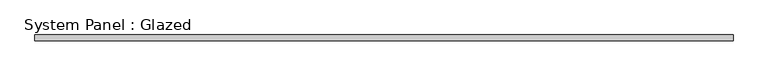
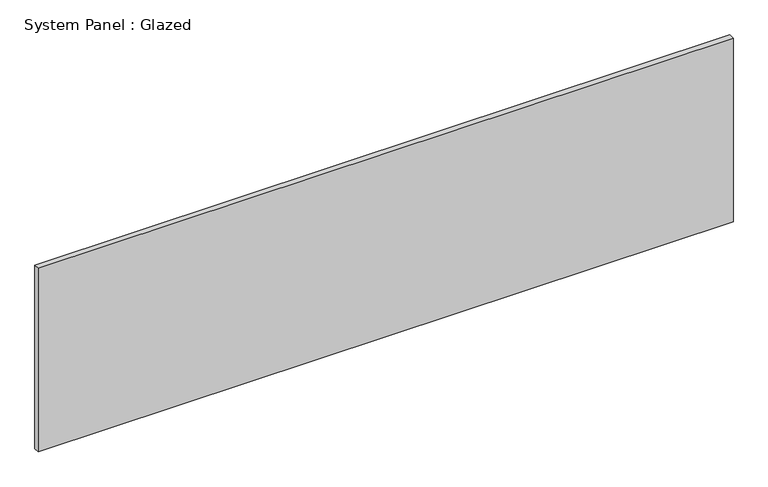
"""IFC4 building model written with IfcOpenShell, lengths in millimetres: plate geometry, System Panel : Glazed."""

import ifcopenshell
import ifcopenshell.guid

model = None  # the IFC model being written
_history = None  # IfcOwnerHistory: only IFC2X3 demands one
_inside = {}  # id of a spatial element -> (the spatial element, [elements in it])
_under = {}  # id of a project, library or spatial element -> (it, [spatial elements below it])
_declared = {}  # id of a project -> (the project, [libraries it declares])
_typed = {}  # id of a type object -> (the type object, [elements of that type])
_made_of = {}  # id of a material, layer set ... -> (it, [elements and type objects made of it])


def new_model(schema):
    """Start an empty IFC model of exactly this schema.

    Asked for "IFC4X3", IfcOpenShell would pick the latest addendum, in which some entities
    have other attributes; the version numbers below select the first issue.
    IFC2X3 requires an IfcOwnerHistory on every rooted entity: one is made here for all.
    """
    global model, _history
    if schema == "IFC4X3":
        model = ifcopenshell.file(schema_version=(4, 3, 0, 0))
    else:
        model = ifcopenshell.file(schema=schema)
    _inside.clear()
    _under.clear()
    _declared.clear()
    _typed.clear()
    _made_of.clear()
    _history = None
    if model.schema == "IFC2X3":
        org = make("IfcOrganization", Name="unknown")
        user = make(
            "IfcPersonAndOrganization",
            ThePerson=make("IfcPerson", FamilyName="unknown"),
            TheOrganization=org,
        )
        app = make(
            "IfcApplication",
            ApplicationDeveloper=org,
            Version="unknown",
            ApplicationFullName="unknown",
            ApplicationIdentifier="unknown",
        )
        _history = make(
            "IfcOwnerHistory",
            OwningUser=user,
            OwningApplication=app,
            ChangeAction="ADDED",
            CreationDate=0,
        )
    return model


def make(cls, **values):
    """One entity of the class cls with the attributes given. An attribute that is None is left unset."""
    return model.create_entity(
        cls, **{name: value for name, value in values.items() if value is not None}
    )


def rooted(cls, **values):
    """An entity with a GlobalId (a new one), such as an element, a storey or a relation."""
    return make(cls, GlobalId=ifcopenshell.guid.new(), OwnerHistory=_history, **values)


def si_unit(unit_type, name, prefix=None):
    """IfcSIUnit, for example si_unit("LENGTHUNIT", "METRE", prefix="MILLI")."""
    return make("IfcSIUnit", UnitType=unit_type, Prefix=prefix, Name=name)


def assignment(units):
    """IfcUnitAssignment: the units of a project."""
    return None if units is None else make("IfcUnitAssignment", Units=units)


def point(xyz):
    """IfcCartesianPoint."""
    return None if xyz is None else make("IfcCartesianPoint", Coordinates=xyz)


def direction(xyz):
    """IfcDirection."""
    return None if xyz is None else make("IfcDirection", DirectionRatios=xyz)


def frame(location, z_axis=None, x_axis=None):
    """IfcAxis2Placement3D, a coordinate frame: its origin and axes. An axis left out is left unset."""
    return make(
        "IfcAxis2Placement3D",
        Location=point(location),
        Axis=direction(z_axis),
        RefDirection=direction(x_axis),
    )


def origin():
    """The frame at (0, 0, 0) with its axes left unset."""
    return frame((0.0, 0.0, 0.0))


def origin_with_axes():
    """The frame at (0, 0, 0) with the z axis (0, 0, 1) and the x axis (1, 0, 0) written out."""
    return frame((0.0, 0.0, 0.0), z_axis=(0.0, 0.0, 1.0), x_axis=(1.0, 0.0, 0.0))


def place(relative_to, where):
    """IfcLocalPlacement: puts the frame where relative to a parent placement (None: the world)."""
    return make(
        "IfcLocalPlacement", PlacementRelTo=relative_to, RelativePlacement=where
    )


def context(
    kind, dimensions, precision=None, world=None, true_north=None, identifier=None
):
    """IfcGeometricRepresentationContext, for example the 3D "Model" context."""
    return make(
        "IfcGeometricRepresentationContext",
        ContextIdentifier=identifier,
        ContextType=kind,
        CoordinateSpaceDimension=dimensions,
        Precision=precision,
        WorldCoordinateSystem=world,
        TrueNorth=true_north,
    )


def project(units=None, contexts=None):
    """IfcProject with its units and contexts."""
    return rooted(
        "IfcProject",
        Name="project",
        RepresentationContexts=contexts,
        UnitsInContext=assignment(units),
    )


def spatial(cls, under=None, at=None, **own):
    """A site, building, storey or space (cls), placed at a placement, below another one or the project."""
    s = rooted(cls, ObjectPlacement=at, **own)
    if under is not None:
        _under.setdefault(under.id(), (under, []))[1].append(s)
    return s


def polyline(points):
    """IfcPolyline through the points."""
    return make("IfcPolyline", Points=[point(p) for p in points])


def outline(outer, holes=None, kind="AREA"):
    """IfcArbitraryClosedProfileDef: a profile drawn as a closed curve; with holes, ...WithVoids."""
    if holes is None:
        return make("IfcArbitraryClosedProfileDef", ProfileType=kind, OuterCurve=outer)
    return make(
        "IfcArbitraryProfileDefWithVoids",
        ProfileType=kind,
        OuterCurve=outer,
        InnerCurves=holes,
    )


def extrude(swept, where, along, depth):
    """IfcExtrudedAreaSolid: the profile swept, set in the frame where, extruded along a direction by depth."""
    return make(
        "IfcExtrudedAreaSolid",
        SweptArea=swept,
        Position=where,
        ExtrudedDirection=direction(along),
        Depth=depth,
    )


def shape(context_of_items, identifier, shape_type, items):
    """IfcShapeRepresentation: the items that make up one representation, for example the "Body"."""
    return make(
        "IfcShapeRepresentation",
        ContextOfItems=context_of_items,
        RepresentationIdentifier=identifier,
        RepresentationType=shape_type,
        Items=items,
    )


def source(mapping_origin, context_of_items, identifier, shape_type, items):
    """IfcRepresentationMap: a shape defined once, which mapped items show again and again."""
    return make(
        "IfcRepresentationMap",
        MappingOrigin=mapping_origin,
        MappedRepresentation=shape(context_of_items, identifier, shape_type, items),
    )


def transform(
    local_origin,
    x_axis=None,
    y_axis=None,
    z_axis=None,
    scale=None,
    scale2=None,
    scale3=None,
    uniform=True,
):
    """IfcCartesianTransformationOperator3D, or its non-uniform kind. x_axis, y_axis, z_axis: its Axis1, 2, 3."""
    if uniform:
        return make(
            "IfcCartesianTransformationOperator3D",
            Axis1=direction(x_axis),
            Axis2=direction(y_axis),
            LocalOrigin=point(local_origin),
            Scale=scale,
            Axis3=direction(z_axis),
        )
    return make(
        "IfcCartesianTransformationOperator3DnonUniform",
        Axis1=direction(x_axis),
        Axis2=direction(y_axis),
        LocalOrigin=point(local_origin),
        Scale=scale,
        Axis3=direction(z_axis),
        Scale2=scale2,
        Scale3=scale3,
    )


def mapped(mapping_source, mapping_target):
    """IfcMappedItem: shows the shape of a source again, moved by a transform."""
    return make(
        "IfcMappedItem", MappingSource=mapping_source, MappingTarget=mapping_target
    )


def made_of(thing, what):
    """Note that an element or type object is made of a material, layer set ...; save() writes the relation."""
    if what is not None:
        _made_of.setdefault(what.id(), (what, []))[1].append(thing)
    return thing


def element(
    cls,
    number,
    at=None,
    inside=None,
    cuts=None,
    type_object=None,
    material=None,
    context=None,
    identifier="Body",
    shape_type=None,
    held_by="IfcProductDefinitionShape",
    body=None,
    shapes=None,
    **own,
):
    """One element of the class cls, such as IfcWall. Its Tag is "e" and its number.

    at: its placement. inside: the storey or other place that contains it. cuts: it is an
    opening in that element (IfcRelVoidsElement). A single representation is given by context,
    identifier, shape_type and body (its items); several are given by shapes. held_by: the class
    of the entity that holds the representations. save() writes the other relations.
    """
    e = rooted(cls, Tag="e%d" % number, ObjectPlacement=at, **own)
    if body is not None:
        shapes = [shape(context, identifier, shape_type, body)]
    if shapes is not None:
        e.Representation = make(held_by, Representations=shapes)
    if inside is not None:
        _inside.setdefault(inside.id(), (inside, []))[1].append(e)
    if cuts is not None:
        rooted(
            "IfcRelVoidsElement", RelatingBuildingElement=cuts, RelatedOpeningElement=e
        )
    if type_object is not None:
        _typed.setdefault(type_object.id(), (type_object, []))[1].append(e)
    return made_of(e, material)


def aggregate(whole, parts):
    """IfcRelAggregates: a whole, such as a stair, and the parts it consists of."""
    return rooted("IfcRelAggregates", RelatingObject=whole, RelatedObjects=parts)


def save(model, path):
    """Write the relations noted so far, then the file.

    IfcRelAggregates (storeys below a building ...), IfcRelContainedInSpatialStructure (elements
    in a storey), IfcRelDefinesByType, IfcRelAssociatesMaterial and IfcRelDeclares: one each for
    every whole, place, type object, material and project.
    """
    for whole, parts in _under.values():
        aggregate(whole, parts)
    for where, things in _inside.values():
        rooted(
            "IfcRelContainedInSpatialStructure",
            RelatedElements=things,
            RelatingStructure=where,
        )
    for kind, things in _typed.values():
        rooted("IfcRelDefinesByType", RelatedObjects=things, RelatingType=kind)
    for what, things in _made_of.values():
        rooted("IfcRelAssociatesMaterial", RelatedObjects=things, RelatingMaterial=what)
    for by, libraries in _declared.values():
        rooted("IfcRelDeclares", RelatingContext=by, RelatedDefinitions=libraries)
    model.write(path)


def system_panel_glazed_8bf11259(model_context):
    return source(origin(), model_context, "Body", "SweptSolid", [
        extrude(outline(polyline([(1549.4, -44.45), (-1549.4, -44.45), (-1549.4, -19.05), (1549.4, -19.05), (1549.4, -44.45)])), origin_with_axes(), (0.0, 0.0, 1.0), 866.0018549),
    ])


if __name__ == "__main__":
    model = new_model("IFC4")
    model_context = context("Model", 3, world=origin())
    ifc_project = project(units=[si_unit("LENGTHUNIT", "METRE", prefix="MILLI")], contexts=[model_context])
    site = spatial("IfcSite", under=ifc_project)
    building = spatial("IfcBuilding", under=site)
    placement = place(None, origin())
    system_panel_glazed_shape = system_panel_glazed_8bf11259(model_context)
    element("IfcPlate", 1, ObjectType="System Panel : Glazed", at=placement, inside=building, context=model_context, shape_type="MappedRepresentation", body=[
        mapped(system_panel_glazed_shape, transform((0.0, 0.0, 0.0), x_axis=(1.0, 0.0, 0.0), y_axis=(0.0, 1.0, 0.0), z_axis=(0.0, 0.0, 1.0))),
    ])
    save(model, "model.ifc")

# Revit data of these elements
# Type "System Panel : Glazed"
#   Construction Type Id = "GSP4R"
#   Analytic Construction = "1/8 in Pilkington single glazing"
#   Visual Light Transmittance = 0.9
#   Solar Heat Gain Coefficient = 0.86
#   Heat Transfer Coefficient (U) = 1.18115 BTU/(h·ft²·°F)
#   Define Thermal Properties by = 1
# Element 1 (IfcPlate, "System Panel : Glazed")
#   Materials on its faces: "Glass"
# Materials
#   "Glass": class "Glass", colour RGB 0 128 192, transparency 0.75, Description = "Soda Lime Glass", Cost = 0
